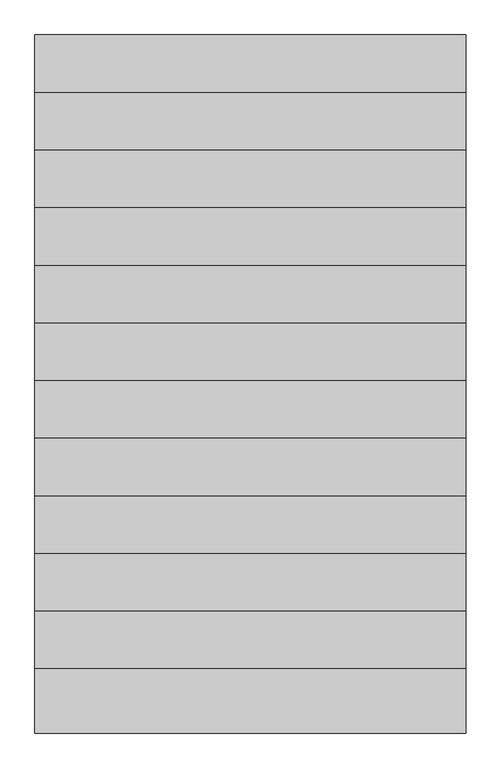
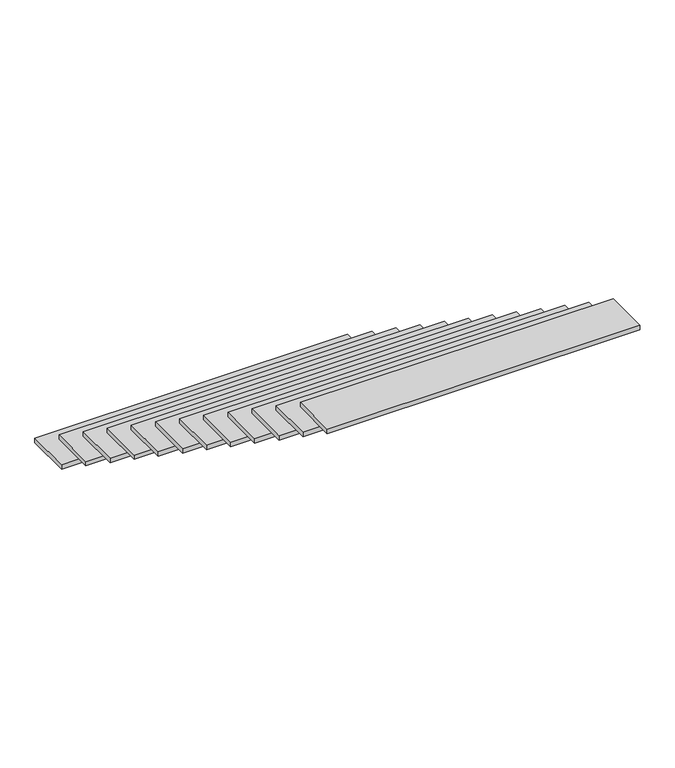
"""IFC4 building model written with IfcOpenShell, lengths in millimetres: stair flight geometry."""

from ifc_helpers import new_model, si_unit, frame, origin, place, context, project, spatial, polyline, outline, extrude, source, transform, mapped, element, save


def stair_flight_1a3f41c4(model_context):
    return source(origin(), model_context, "Body", "SweptSolid", [
        extrude(outline(polyline([(6057.6628143, 4368.4492804), (4057.6628143, 4368.4492804), (4057.6628143, 4665.6409511), (6057.6628143, 4665.6409511), (6057.6628143, 4368.4492804)])), frame((0.0, 0.0, -1406.0958353), z_axis=(0.0, 0.0, 1.0), x_axis=(1.0, 0.0, 0.0)), (0.0, 0.0, 1.0), 30.0),
        extrude(outline(polyline([(6057.6628143, 4101.2576098), (4057.6628143, 4101.2576098), (4057.6628143, 4398.4492804), (6057.6628143, 4398.4492804), (6057.6628143, 4101.2576098)])), frame((0.0, 0.0, -1222.1916707), z_axis=(0.0, 0.0, 1.0), x_axis=(1.0, 0.0, 0.0)), (0.0, 0.0, 1.0), 30.0),
        extrude(outline(polyline([(6057.6628143, 3834.0659391), (4057.6628143, 3834.0659391), (4057.6628143, 4131.2576098), (6057.6628143, 4131.2576098), (6057.6628143, 3834.0659391)])), frame((0.0, 0.0, -1038.287506), z_axis=(0.0, 0.0, 1.0), x_axis=(1.0, 0.0, 0.0)), (0.0, 0.0, 1.0), 30.0),
        extrude(outline(polyline([(6057.6628143, 3566.8742684), (4057.6628143, 3566.8742684), (4057.6628143, 3864.0659391), (6057.6628143, 3864.0659391), (6057.6628143, 3566.8742684)])), frame((0.0, 0.0, -854.3833413), z_axis=(0.0, 0.0, 1.0), x_axis=(1.0, 0.0, 0.0)), (0.0, 0.0, 1.0), 30.0),
        extrude(outline(polyline([(6057.6628143, 3299.6825978), (4057.6628143, 3299.6825978), (4057.6628143, 3596.8742684), (6057.6628143, 3596.8742684), (6057.6628143, 3299.6825978)])), frame((0.0, 0.0, -670.4791766), z_axis=(0.0, 0.0, 1.0), x_axis=(1.0, 0.0, 0.0)), (0.0, 0.0, 1.0), 30.0),
        extrude(outline(polyline([(6057.6628143, 3032.4909271), (4057.6628143, 3032.4909271), (4057.6628143, 3329.6825978), (6057.6628143, 3329.6825978), (6057.6628143, 3032.4909271)])), frame((0.0, 0.0, -486.575012), z_axis=(0.0, 0.0, 1.0), x_axis=(1.0, 0.0, 0.0)), (0.0, 0.0, 1.0), 30.0),
        extrude(outline(polyline([(6057.6628143, 2765.2992565), (4057.6628143, 2765.2992565), (4057.6628143, 3062.4909271), (6057.6628143, 3062.4909271), (6057.6628143, 2765.2992565)])), frame((0.0, 0.0, -302.6708473), z_axis=(0.0, 0.0, 1.0), x_axis=(1.0, 0.0, 0.0)), (0.0, 0.0, 1.0), 30.0),
        extrude(outline(polyline([(6057.6628143, 2498.1075858), (4057.6628143, 2498.1075858), (4057.6628143, 2795.2992565), (6057.6628143, 2795.2992565), (6057.6628143, 2498.1075858)])), frame((0.0, 0.0, -118.7666826), z_axis=(0.0, 0.0, 1.0), x_axis=(1.0, 0.0, 0.0)), (0.0, 0.0, 1.0), 30.0),
        extrude(outline(polyline([(6057.6628143, 2230.9159152), (4057.6628143, 2230.9159152), (4057.6628143, 2528.1075858), (6057.6628143, 2528.1075858), (6057.6628143, 2230.9159152)])), frame((0.0, 0.0, 65.137482), z_axis=(0.0, 0.0, 1.0), x_axis=(1.0, 0.0, 0.0)), (0.0, 0.0, 1.0), 30.0),
        extrude(outline(polyline([(6057.6628143, 1963.7242445), (4057.6628143, 1963.7242445), (4057.6628143, 2260.9159152), (6057.6628143, 2260.9159152), (6057.6628143, 1963.7242445)])), frame((0.0, 0.0, 249.0416467), z_axis=(0.0, 0.0, 1.0), x_axis=(1.0, 0.0, 0.0)), (0.0, 0.0, 1.0), 30.0),
        extrude(outline(polyline([(6057.6628143, 1696.5325738), (4057.6628143, 1696.5325738), (4057.6628143, 1993.7242445), (6057.6628143, 1993.7242445), (6057.6628143, 1696.5325738)])), frame((0.0, 0.0, 432.9458114), z_axis=(0.0, 0.0, 1.0), x_axis=(1.0, 0.0, 0.0)), (0.0, 0.0, 1.0), 30.0),
        extrude(outline(polyline([(6057.6628143, 1429.3409032), (4057.6628143, 1429.3409032), (4057.6628143, 1726.5325738), (6057.6628143, 1726.5325738), (6057.6628143, 1429.3409032)])), frame((0.0, 0.0, 616.8499761), z_axis=(0.0, 0.0, 1.0), x_axis=(1.0, 0.0, 0.0)), (0.0, 0.0, 1.0), 30.0),
    ])


if __name__ == "__main__":
    model = new_model("IFC4")
    model_context = context("Model", 3, world=origin())
    ifc_project = project(units=[si_unit("LENGTHUNIT", "METRE", prefix="MILLI")], contexts=[model_context])
    site = spatial("IfcSite", under=ifc_project)
    building = spatial("IfcBuilding", under=site)
    placement = place(None, origin())
    stair_flight_shape = stair_flight_1a3f41c4(model_context)
    element("IfcStairFlight", 1, at=placement, inside=building, context=model_context, shape_type="MappedRepresentation", body=[
        mapped(stair_flight_shape, transform((0.0, 0.0, 0.0), x_axis=(1.0, 0.0, 0.0), y_axis=(0.0, 1.0, 0.0), z_axis=(0.0, 0.0, 1.0))),
    ])
    save(model, "model.ifc")

# Revit data of these elements
# Element 1 (IfcStairFlight)
#   Materials on its faces: "Standard - Treppe"
# Materials
#   "Standard - Treppe": class "Allgemeines", colour RGB 128 128 128, transparency 0, Cost = 0
